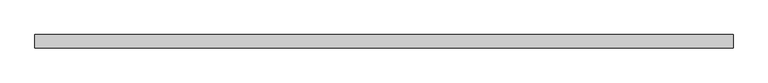
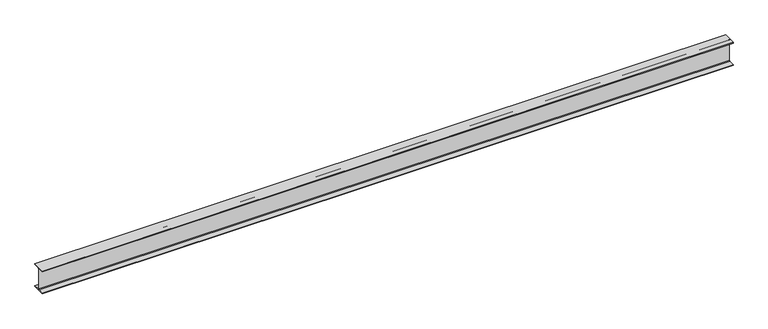
"""IFC4 building model written with IfcOpenShell, lengths in millimetres: beam geometry, Old_Steel Beam_H-KSD3502 : H_SB_ASB_H-488×300x11x18."""

from ifc_helpers import new_model, si_unit, point, frame, frame_2d, origin, place, context, project, spatial, polyline, circle_curve, trimmed, segment, composite_curve, outline, extrude, source, transform, mapped, element, save


def beam_db5af9cf(model_context):
    return source(origin(), model_context, "Body", "SweptSolid", [
        extrude(outline(composite_curve([segment(polyline([(82.5, -141.5), (82.5, -151.7), (-82.5, -151.7), (-82.5, -141.5), (-11.9, -141.5)]), True, "CONTINUOUS"), segment(trimmed(circle_curve(frame_2d((-11.9, -132.6)), 8.9), [point((-11.9, -141.5))], [point((-3.0, -132.6))], True, "CARTESIAN"), True, "CONTINUOUS"), segment(polyline([(-3.0, -132.6), (-3.0, 132.6)]), True, "CONTINUOUS"), segment(trimmed(circle_curve(frame_2d((-11.9, 132.6)), 8.9), [point((-3.0, 132.6))], [point((-11.9, 141.5))], True, "CARTESIAN"), True, "CONTINUOUS"), segment(polyline([(-11.9, 141.5), (-82.5, 141.5), (-82.5, 151.7), (82.5, 151.7), (82.5, 141.5), (11.9, 141.5)]), True, "CONTINUOUS"), segment(trimmed(circle_curve(frame_2d((11.9, 132.6)), 8.9), [point((11.9, 141.5))], [point((3.0, 132.6))], True, "CARTESIAN"), True, "CONTINUOUS"), segment(polyline([(3.0, 132.6), (3.0, -132.6)]), True, "CONTINUOUS"), segment(trimmed(circle_curve(frame_2d((11.9, -132.6)), 8.9), [point((3.0, -132.6))], [point((11.9, -141.5))], True, "CARTESIAN"), True, "CONTINUOUS"), segment(polyline([(11.9, -141.5), (82.5, -141.5)]), True, "CONTINUOUS")], self_intersect=False)), frame((-4337.3, 0.0, 0.0), z_axis=(1.0, 0.0, 0.0), x_axis=(0.0, 1.0, 0.0)), (0.0, 0.0, 1.0), 8674.6),
    ])


if __name__ == "__main__":
    model = new_model("IFC4")
    model_context = context("Model", 3, world=origin())
    ifc_project = project(units=[si_unit("LENGTHUNIT", "METRE", prefix="MILLI")], contexts=[model_context])
    site = spatial("IfcSite", under=ifc_project)
    building = spatial("IfcBuilding", under=site)
    placement = place(None, origin())
    beam_shape = beam_db5af9cf(model_context)
    element("IfcBeam", 1, ObjectType="Old_Steel Beam_H-KSD3502 : H_SB_ASB_H-488×300x11x18", at=placement, inside=building, context=model_context, shape_type="MappedRepresentation", body=[
        mapped(beam_shape, transform((0.0, 0.0, 0.0), x_axis=(1.0, 0.0, 0.0), y_axis=(0.0, 1.0, 0.0), z_axis=(0.0, 0.0, 1.0))),
    ])
    save(model, "model.ifc")

# Revit data of these elements
# Type "Old_Steel Beam_H-KSD3502 : H_SB_ASB_H-488×300x11x18"
#   Width = 30.0 cm
#   Web Thickness = 1.1 cm
#   Web Fillet = 2.6 cm
#   Warping Constant = 4473230.0 cm⁶
#   Torsional Moment of Inertia = 137.492 cm⁴
#   Torsional Modulus = 1.0 cm³
#   Section Area = 163.5 cm²
#   Plastic Modulus weak axis = 830.0 cm³
#   Plastic Modulus strong axis = 3230.0 cm³
#   Perimeter = 2.11 m²/m
#   Nominal Weight = 128.00 kgf/m
#   Moment of Inertia weak axis = 8110.00 cm⁴
#   Moment of Inertia strong axis = 71000.00 cm⁴
#   Height = 48.8 cm
#   Flange Thickness = 1.8 cm
#   Elastic Modulus weak axis = 541.0 cm³
#   Elastic Modulus strong axis = 2910.0 cm³
#   Centroid Vertical = 24.4 cm
#   Centroid Horizontal = 15.0 cm
#   Length [instance default] = 1.5240 m
#   Structural Material [instance default] = Steel, 45-345
#   Assembly Code = ""
# Element 1 (IfcBeam, "Old_Steel Beam_H-KSD3502 : H_SB_ASB_H-488×300x11x18")
#   Structural Material = none
# Materials
#   "Steel, 45-345": class "Metal", colour RGB 189 187 185, transparency 0, Description = "Steel 345 MPa", Cost = 0
